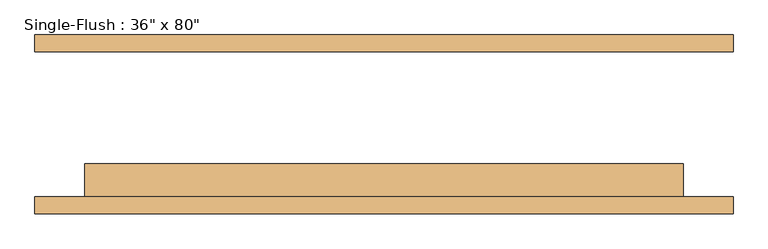
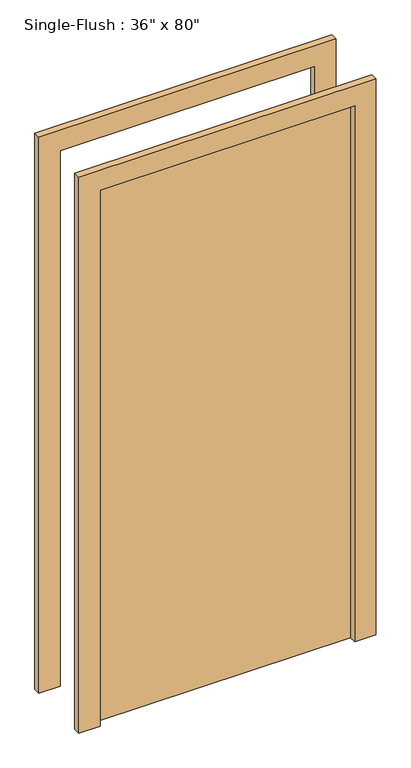
"""IFC4 building model written with IfcOpenShell, lengths in millimetres: door geometry."""

import ifcopenshell
import ifcopenshell.guid

model = None  # the IFC model being written
_history = None  # IfcOwnerHistory: only IFC2X3 demands one
_inside = {}  # id of a spatial element -> (the spatial element, [elements in it])
_under = {}  # id of a project, library or spatial element -> (it, [spatial elements below it])
_declared = {}  # id of a project -> (the project, [libraries it declares])
_typed = {}  # id of a type object -> (the type object, [elements of that type])
_made_of = {}  # id of a material, layer set ... -> (it, [elements and type objects made of it])


def new_model(schema):
    """Start an empty IFC model of exactly this schema.

    Asked for "IFC4X3", IfcOpenShell would pick the latest addendum, in which some entities
    have other attributes; the version numbers below select the first issue.
    IFC2X3 requires an IfcOwnerHistory on every rooted entity: one is made here for all.
    """
    global model, _history
    if schema == "IFC4X3":
        model = ifcopenshell.file(schema_version=(4, 3, 0, 0))
    else:
        model = ifcopenshell.file(schema=schema)
    _inside.clear()
    _under.clear()
    _declared.clear()
    _typed.clear()
    _made_of.clear()
    _history = None
    if model.schema == "IFC2X3":
        org = make("IfcOrganization", Name="unknown")
        user = make(
            "IfcPersonAndOrganization",
            ThePerson=make("IfcPerson", FamilyName="unknown"),
            TheOrganization=org,
        )
        app = make(
            "IfcApplication",
            ApplicationDeveloper=org,
            Version="unknown",
            ApplicationFullName="unknown",
            ApplicationIdentifier="unknown",
        )
        _history = make(
            "IfcOwnerHistory",
            OwningUser=user,
            OwningApplication=app,
            ChangeAction="ADDED",
            CreationDate=0,
        )
    return model


def make(cls, **values):
    """One entity of the class cls with the attributes given. An attribute that is None is left unset."""
    return model.create_entity(
        cls, **{name: value for name, value in values.items() if value is not None}
    )


def rooted(cls, **values):
    """An entity with a GlobalId (a new one), such as an element, a storey or a relation."""
    return make(cls, GlobalId=ifcopenshell.guid.new(), OwnerHistory=_history, **values)


def si_unit(unit_type, name, prefix=None):
    """IfcSIUnit, for example si_unit("LENGTHUNIT", "METRE", prefix="MILLI")."""
    return make("IfcSIUnit", UnitType=unit_type, Prefix=prefix, Name=name)


def assignment(units):
    """IfcUnitAssignment: the units of a project."""
    return None if units is None else make("IfcUnitAssignment", Units=units)


def point(xyz):
    """IfcCartesianPoint."""
    return None if xyz is None else make("IfcCartesianPoint", Coordinates=xyz)


def direction(xyz):
    """IfcDirection."""
    return None if xyz is None else make("IfcDirection", DirectionRatios=xyz)


def frame(location, z_axis=None, x_axis=None):
    """IfcAxis2Placement3D, a coordinate frame: its origin and axes. An axis left out is left unset."""
    return make(
        "IfcAxis2Placement3D",
        Location=point(location),
        Axis=direction(z_axis),
        RefDirection=direction(x_axis),
    )


def origin():
    """The frame at (0, 0, 0) with its axes left unset."""
    return frame((0.0, 0.0, 0.0))


def origin_with_axes():
    """The frame at (0, 0, 0) with the z axis (0, 0, 1) and the x axis (1, 0, 0) written out."""
    return frame((0.0, 0.0, 0.0), z_axis=(0.0, 0.0, 1.0), x_axis=(1.0, 0.0, 0.0))


def place(relative_to, where):
    """IfcLocalPlacement: puts the frame where relative to a parent placement (None: the world)."""
    return make(
        "IfcLocalPlacement", PlacementRelTo=relative_to, RelativePlacement=where
    )


def context(
    kind, dimensions, precision=None, world=None, true_north=None, identifier=None
):
    """IfcGeometricRepresentationContext, for example the 3D "Model" context."""
    return make(
        "IfcGeometricRepresentationContext",
        ContextIdentifier=identifier,
        ContextType=kind,
        CoordinateSpaceDimension=dimensions,
        Precision=precision,
        WorldCoordinateSystem=world,
        TrueNorth=true_north,
    )


def project(units=None, contexts=None):
    """IfcProject with its units and contexts."""
    return rooted(
        "IfcProject",
        Name="project",
        RepresentationContexts=contexts,
        UnitsInContext=assignment(units),
    )


def spatial(cls, under=None, at=None, **own):
    """A site, building, storey or space (cls), placed at a placement, below another one or the project."""
    s = rooted(cls, ObjectPlacement=at, **own)
    if under is not None:
        _under.setdefault(under.id(), (under, []))[1].append(s)
    return s


def polyline(points):
    """IfcPolyline through the points."""
    return make("IfcPolyline", Points=[point(p) for p in points])


def outline(outer, holes=None, kind="AREA"):
    """IfcArbitraryClosedProfileDef: a profile drawn as a closed curve; with holes, ...WithVoids."""
    if holes is None:
        return make("IfcArbitraryClosedProfileDef", ProfileType=kind, OuterCurve=outer)
    return make(
        "IfcArbitraryProfileDefWithVoids",
        ProfileType=kind,
        OuterCurve=outer,
        InnerCurves=holes,
    )


def extrude(swept, where, along, depth):
    """IfcExtrudedAreaSolid: the profile swept, set in the frame where, extruded along a direction by depth."""
    return make(
        "IfcExtrudedAreaSolid",
        SweptArea=swept,
        Position=where,
        ExtrudedDirection=direction(along),
        Depth=depth,
    )


def shape(context_of_items, identifier, shape_type, items):
    """IfcShapeRepresentation: the items that make up one representation, for example the "Body"."""
    return make(
        "IfcShapeRepresentation",
        ContextOfItems=context_of_items,
        RepresentationIdentifier=identifier,
        RepresentationType=shape_type,
        Items=items,
    )


def source(mapping_origin, context_of_items, identifier, shape_type, items):
    """IfcRepresentationMap: a shape defined once, which mapped items show again and again."""
    return make(
        "IfcRepresentationMap",
        MappingOrigin=mapping_origin,
        MappedRepresentation=shape(context_of_items, identifier, shape_type, items),
    )


def transform(
    local_origin,
    x_axis=None,
    y_axis=None,
    z_axis=None,
    scale=None,
    scale2=None,
    scale3=None,
    uniform=True,
):
    """IfcCartesianTransformationOperator3D, or its non-uniform kind. x_axis, y_axis, z_axis: its Axis1, 2, 3."""
    if uniform:
        return make(
            "IfcCartesianTransformationOperator3D",
            Axis1=direction(x_axis),
            Axis2=direction(y_axis),
            LocalOrigin=point(local_origin),
            Scale=scale,
            Axis3=direction(z_axis),
        )
    return make(
        "IfcCartesianTransformationOperator3DnonUniform",
        Axis1=direction(x_axis),
        Axis2=direction(y_axis),
        LocalOrigin=point(local_origin),
        Scale=scale,
        Axis3=direction(z_axis),
        Scale2=scale2,
        Scale3=scale3,
    )


def mapped(mapping_source, mapping_target):
    """IfcMappedItem: shows the shape of a source again, moved by a transform."""
    return make(
        "IfcMappedItem", MappingSource=mapping_source, MappingTarget=mapping_target
    )


def made_of(thing, what):
    """Note that an element or type object is made of a material, layer set ...; save() writes the relation."""
    if what is not None:
        _made_of.setdefault(what.id(), (what, []))[1].append(thing)
    return thing


def element(
    cls,
    number,
    at=None,
    inside=None,
    cuts=None,
    type_object=None,
    material=None,
    context=None,
    identifier="Body",
    shape_type=None,
    held_by="IfcProductDefinitionShape",
    body=None,
    shapes=None,
    **own,
):
    """One element of the class cls, such as IfcWall. Its Tag is "e" and its number.

    at: its placement. inside: the storey or other place that contains it. cuts: it is an
    opening in that element (IfcRelVoidsElement). A single representation is given by context,
    identifier, shape_type and body (its items); several are given by shapes. held_by: the class
    of the entity that holds the representations. save() writes the other relations.
    """
    e = rooted(cls, Tag="e%d" % number, ObjectPlacement=at, **own)
    if body is not None:
        shapes = [shape(context, identifier, shape_type, body)]
    if shapes is not None:
        e.Representation = make(held_by, Representations=shapes)
    if inside is not None:
        _inside.setdefault(inside.id(), (inside, []))[1].append(e)
    if cuts is not None:
        rooted(
            "IfcRelVoidsElement", RelatingBuildingElement=cuts, RelatedOpeningElement=e
        )
    if type_object is not None:
        _typed.setdefault(type_object.id(), (type_object, []))[1].append(e)
    return made_of(e, material)


def aggregate(whole, parts):
    """IfcRelAggregates: a whole, such as a stair, and the parts it consists of."""
    return rooted("IfcRelAggregates", RelatingObject=whole, RelatedObjects=parts)


def save(model, path):
    """Write the relations noted so far, then the file.

    IfcRelAggregates (storeys below a building ...), IfcRelContainedInSpatialStructure (elements
    in a storey), IfcRelDefinesByType, IfcRelAssociatesMaterial and IfcRelDeclares: one each for
    every whole, place, type object, material and project.
    """
    for whole, parts in _under.values():
        aggregate(whole, parts)
    for where, things in _inside.values():
        rooted(
            "IfcRelContainedInSpatialStructure",
            RelatedElements=things,
            RelatingStructure=where,
        )
    for kind, things in _typed.values():
        rooted("IfcRelDefinesByType", RelatedObjects=things, RelatingType=kind)
    for what, things in _made_of.values():
        rooted("IfcRelAssociatesMaterial", RelatedObjects=things, RelatingMaterial=what)
    for by, libraries in _declared.values():
        rooted("IfcRelDeclares", RelatingContext=by, RelatedDefinitions=libraries)
    model.write(path)


def door_d5b76e51(model_context):
    return source(origin(), model_context, "Body", "SweptSolid", [
        extrude(outline(polyline([(2108.2, -533.4), (0.0, -533.4), (0.0, -457.2), (2032.0, -457.2), (2032.0, 457.2), (0.0, 457.2), (0.0, 533.4), (2108.2, 533.4), (2108.2, -533.4)])), frame((0.0, -136.525, 0.0), z_axis=(0.0, 1.0, 0.0), x_axis=(0.0, 0.0, 1.0)), (0.0, 0.0, 1.0), 25.4),
        extrude(outline(polyline([(2108.2, 533.4), (2108.2, -533.4), (0.0, -533.4), (0.0, -457.2), (2032.0, -457.2), (2032.0, 457.2), (0.0, 457.2), (0.0, 533.4), (2108.2, 533.4)])), frame((0.0, 111.125, 0.0), z_axis=(0.0, 1.0, 0.0), x_axis=(0.0, 0.0, 1.0)), (0.0, 0.0, 1.0), 25.4),
        extrude(outline(polyline([(457.2, -60.325), (457.2, -111.125), (-457.2, -111.125), (-457.2, -60.325), (457.2, -60.325)])), origin_with_axes(), (0.0, 0.0, 1.0), 2032.0),
    ])


if __name__ == "__main__":
    model = new_model("IFC4")
    model_context = context("Model", 3, world=origin())
    ifc_project = project(units=[si_unit("LENGTHUNIT", "METRE", prefix="MILLI")], contexts=[model_context])
    site = spatial("IfcSite", under=ifc_project)
    building = spatial("IfcBuilding", under=site)
    placement = place(None, origin())
    door_shape = door_d5b76e51(model_context)
    element("IfcDoor", 1, ObjectType="Single-Flush : 36\" x 80\"", at=placement, inside=building, context=model_context, shape_type="MappedRepresentation", body=[
        mapped(door_shape, transform((0.0, 0.0, 0.0), x_axis=(1.0, 0.0, 0.0), y_axis=(0.0, 1.0, 0.0), z_axis=(0.0, 0.0, 1.0))),
    ])
    save(model, "model.ifc")

# Revit data of these elements
# Type "Single-Flush : 36\" x 80\""
#   Type Mark = "13"
#   Construction Type Id = "MDOOR"
#   Assembly Code = "C1020"
#   Analytic Construction = "Metal"
#   Thickness = 0' - 2"
#   Heat Transfer Coefficient (U) = 3.7021 W/(m²·K)
#   Height = 6' - 8"
#   Trim Projection Ext = 0' - 1"
#   Trim Projection Int = 0' - 1"
#   Trim Width = 0' - 3"
#   Width = 3' - 0"
#   Door Material = INTERIOR GRADE ALUMINUM STOREFRONT W/ SAFETY GLAZING
#   Frame Material = INTERIOR GRADE ALUMINUM STOREFRONT W/ SAFETY GLAZING
#   Visual Light Transmittance = 0
#   Solar Heat Gain Coefficient = 0
#   Function = (empty or 0)
#   Wall Closure = (empty or 0)
# Element 1 (IfcDoor, "Single-Flush : 36\" x 80\"")
#   Materials on its faces: "INTERIOR GRADE ALUMINUM STOREFRONT W/ SAFETY GLAZING"
# Materials
#   "INTERIOR GRADE ALUMINUM STOREFRONT W/ SAFETY GLAZING": class "Metal", colour RGB 226 226 226, transparency 0, Description = "Aluminum 6061", Cost = 0
